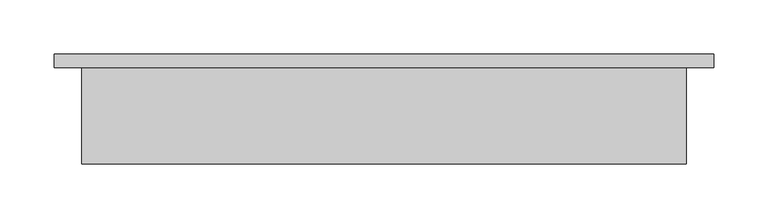
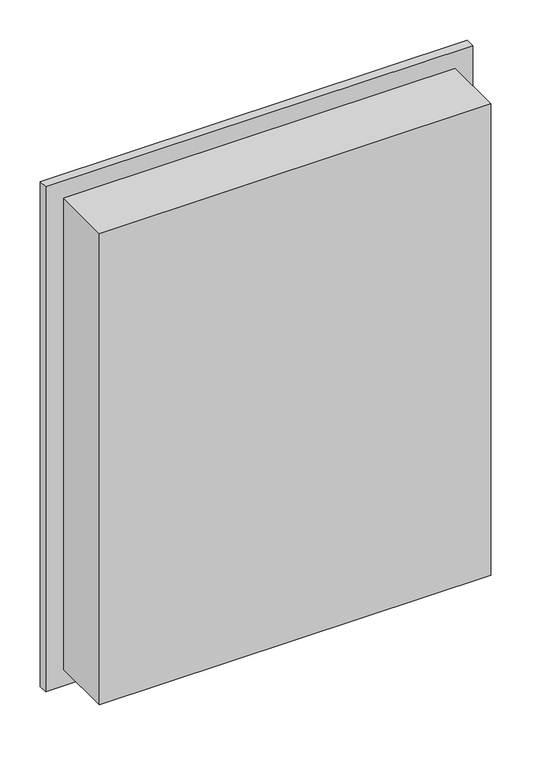
"""IFC4 building model written with IfcOpenShell, lengths in millimetres: furniture geometry, Medicine Cabinet, Recessed-NON-COLLECTUS : -."""

import ifcopenshell
import ifcopenshell.guid

model = None  # the IFC model being written
_history = None  # IfcOwnerHistory: only IFC2X3 demands one
_inside = {}  # id of a spatial element -> (the spatial element, [elements in it])
_under = {}  # id of a project, library or spatial element -> (it, [spatial elements below it])
_declared = {}  # id of a project -> (the project, [libraries it declares])
_typed = {}  # id of a type object -> (the type object, [elements of that type])
_made_of = {}  # id of a material, layer set ... -> (it, [elements and type objects made of it])


def new_model(schema):
    """Start an empty IFC model of exactly this schema.

    Asked for "IFC4X3", IfcOpenShell would pick the latest addendum, in which some entities
    have other attributes; the version numbers below select the first issue.
    IFC2X3 requires an IfcOwnerHistory on every rooted entity: one is made here for all.
    """
    global model, _history
    if schema == "IFC4X3":
        model = ifcopenshell.file(schema_version=(4, 3, 0, 0))
    else:
        model = ifcopenshell.file(schema=schema)
    _inside.clear()
    _under.clear()
    _declared.clear()
    _typed.clear()
    _made_of.clear()
    _history = None
    if model.schema == "IFC2X3":
        org = make("IfcOrganization", Name="unknown")
        user = make(
            "IfcPersonAndOrganization",
            ThePerson=make("IfcPerson", FamilyName="unknown"),
            TheOrganization=org,
        )
        app = make(
            "IfcApplication",
            ApplicationDeveloper=org,
            Version="unknown",
            ApplicationFullName="unknown",
            ApplicationIdentifier="unknown",
        )
        _history = make(
            "IfcOwnerHistory",
            OwningUser=user,
            OwningApplication=app,
            ChangeAction="ADDED",
            CreationDate=0,
        )
    return model


def make(cls, **values):
    """One entity of the class cls with the attributes given. An attribute that is None is left unset."""
    return model.create_entity(
        cls, **{name: value for name, value in values.items() if value is not None}
    )


def rooted(cls, **values):
    """An entity with a GlobalId (a new one), such as an element, a storey or a relation."""
    return make(cls, GlobalId=ifcopenshell.guid.new(), OwnerHistory=_history, **values)


def si_unit(unit_type, name, prefix=None):
    """IfcSIUnit, for example si_unit("LENGTHUNIT", "METRE", prefix="MILLI")."""
    return make("IfcSIUnit", UnitType=unit_type, Prefix=prefix, Name=name)


def assignment(units):
    """IfcUnitAssignment: the units of a project."""
    return None if units is None else make("IfcUnitAssignment", Units=units)


def point(xyz):
    """IfcCartesianPoint."""
    return None if xyz is None else make("IfcCartesianPoint", Coordinates=xyz)


def direction(xyz):
    """IfcDirection."""
    return None if xyz is None else make("IfcDirection", DirectionRatios=xyz)


def frame(location, z_axis=None, x_axis=None):
    """IfcAxis2Placement3D, a coordinate frame: its origin and axes. An axis left out is left unset."""
    return make(
        "IfcAxis2Placement3D",
        Location=point(location),
        Axis=direction(z_axis),
        RefDirection=direction(x_axis),
    )


def origin():
    """The frame at (0, 0, 0) with its axes left unset."""
    return frame((0.0, 0.0, 0.0))


def place(relative_to, where):
    """IfcLocalPlacement: puts the frame where relative to a parent placement (None: the world)."""
    return make(
        "IfcLocalPlacement", PlacementRelTo=relative_to, RelativePlacement=where
    )


def context(
    kind, dimensions, precision=None, world=None, true_north=None, identifier=None
):
    """IfcGeometricRepresentationContext, for example the 3D "Model" context."""
    return make(
        "IfcGeometricRepresentationContext",
        ContextIdentifier=identifier,
        ContextType=kind,
        CoordinateSpaceDimension=dimensions,
        Precision=precision,
        WorldCoordinateSystem=world,
        TrueNorth=true_north,
    )


def project(units=None, contexts=None):
    """IfcProject with its units and contexts."""
    return rooted(
        "IfcProject",
        Name="project",
        RepresentationContexts=contexts,
        UnitsInContext=assignment(units),
    )


def spatial(cls, under=None, at=None, **own):
    """A site, building, storey or space (cls), placed at a placement, below another one or the project."""
    s = rooted(cls, ObjectPlacement=at, **own)
    if under is not None:
        _under.setdefault(under.id(), (under, []))[1].append(s)
    return s


def polyline(points):
    """IfcPolyline through the points."""
    return make("IfcPolyline", Points=[point(p) for p in points])


def outline(outer, holes=None, kind="AREA"):
    """IfcArbitraryClosedProfileDef: a profile drawn as a closed curve; with holes, ...WithVoids."""
    if holes is None:
        return make("IfcArbitraryClosedProfileDef", ProfileType=kind, OuterCurve=outer)
    return make(
        "IfcArbitraryProfileDefWithVoids",
        ProfileType=kind,
        OuterCurve=outer,
        InnerCurves=holes,
    )


def extrude(swept, where, along, depth):
    """IfcExtrudedAreaSolid: the profile swept, set in the frame where, extruded along a direction by depth."""
    return make(
        "IfcExtrudedAreaSolid",
        SweptArea=swept,
        Position=where,
        ExtrudedDirection=direction(along),
        Depth=depth,
    )


def faces_of(points, faces, orient=None, outer=None):
    """IfcFace entities. A face is a list of loops; a loop is a list of indices into points, from 0.

    orient and outer hold one flag for each loop. By default every Orientation is true, the
    first loop of a face is its IfcFaceOuterBound and the others are IfcFaceBound.
    """
    made = []
    for i, loops in enumerate(faces):
        bounds = []
        for j, loop in enumerate(loops):
            is_outer = j == 0 if outer is None else outer[i][j]
            bounds.append(
                make(
                    "IfcFaceOuterBound" if is_outer else "IfcFaceBound",
                    Bound=make("IfcPolyLoop", Polygon=[points[k] for k in loop]),
                    Orientation=True if orient is None else orient[i][j],
                )
            )
        made.append(make("IfcFace", Bounds=bounds))
    return made


def faceted_brep(points, faces, orient=None, outer=None, voids=None):
    """IfcFacetedBrep: a solid bounded by flat faces; with voids (closed shells), ...WithVoids."""
    shared = [point(p) for p in points]
    hull = make("IfcClosedShell", CfsFaces=faces_of(shared, faces, orient, outer))
    if voids is None:
        return make("IfcFacetedBrep", Outer=hull)
    return make(
        "IfcFacetedBrepWithVoids",
        Outer=hull,
        Voids=[
            make(cls, CfsFaces=faces_of(shared, fs, o, b)) for cls, fs, o, b in voids
        ],
    )


def shape(context_of_items, identifier, shape_type, items):
    """IfcShapeRepresentation: the items that make up one representation, for example the "Body"."""
    return make(
        "IfcShapeRepresentation",
        ContextOfItems=context_of_items,
        RepresentationIdentifier=identifier,
        RepresentationType=shape_type,
        Items=items,
    )


def source(mapping_origin, context_of_items, identifier, shape_type, items):
    """IfcRepresentationMap: a shape defined once, which mapped items show again and again."""
    return make(
        "IfcRepresentationMap",
        MappingOrigin=mapping_origin,
        MappedRepresentation=shape(context_of_items, identifier, shape_type, items),
    )


def transform(
    local_origin,
    x_axis=None,
    y_axis=None,
    z_axis=None,
    scale=None,
    scale2=None,
    scale3=None,
    uniform=True,
):
    """IfcCartesianTransformationOperator3D, or its non-uniform kind. x_axis, y_axis, z_axis: its Axis1, 2, 3."""
    if uniform:
        return make(
            "IfcCartesianTransformationOperator3D",
            Axis1=direction(x_axis),
            Axis2=direction(y_axis),
            LocalOrigin=point(local_origin),
            Scale=scale,
            Axis3=direction(z_axis),
        )
    return make(
        "IfcCartesianTransformationOperator3DnonUniform",
        Axis1=direction(x_axis),
        Axis2=direction(y_axis),
        LocalOrigin=point(local_origin),
        Scale=scale,
        Axis3=direction(z_axis),
        Scale2=scale2,
        Scale3=scale3,
    )


def mapped(mapping_source, mapping_target):
    """IfcMappedItem: shows the shape of a source again, moved by a transform."""
    return make(
        "IfcMappedItem", MappingSource=mapping_source, MappingTarget=mapping_target
    )


def made_of(thing, what):
    """Note that an element or type object is made of a material, layer set ...; save() writes the relation."""
    if what is not None:
        _made_of.setdefault(what.id(), (what, []))[1].append(thing)
    return thing


def element(
    cls,
    number,
    at=None,
    inside=None,
    cuts=None,
    type_object=None,
    material=None,
    context=None,
    identifier="Body",
    shape_type=None,
    held_by="IfcProductDefinitionShape",
    body=None,
    shapes=None,
    **own,
):
    """One element of the class cls, such as IfcWall. Its Tag is "e" and its number.

    at: its placement. inside: the storey or other place that contains it. cuts: it is an
    opening in that element (IfcRelVoidsElement). A single representation is given by context,
    identifier, shape_type and body (its items); several are given by shapes. held_by: the class
    of the entity that holds the representations. save() writes the other relations.
    """
    e = rooted(cls, Tag="e%d" % number, ObjectPlacement=at, **own)
    if body is not None:
        shapes = [shape(context, identifier, shape_type, body)]
    if shapes is not None:
        e.Representation = make(held_by, Representations=shapes)
    if inside is not None:
        _inside.setdefault(inside.id(), (inside, []))[1].append(e)
    if cuts is not None:
        rooted(
            "IfcRelVoidsElement", RelatingBuildingElement=cuts, RelatedOpeningElement=e
        )
    if type_object is not None:
        _typed.setdefault(type_object.id(), (type_object, []))[1].append(e)
    return made_of(e, material)


def aggregate(whole, parts):
    """IfcRelAggregates: a whole, such as a stair, and the parts it consists of."""
    return rooted("IfcRelAggregates", RelatingObject=whole, RelatedObjects=parts)


def save(model, path):
    """Write the relations noted so far, then the file.

    IfcRelAggregates (storeys below a building ...), IfcRelContainedInSpatialStructure (elements
    in a storey), IfcRelDefinesByType, IfcRelAssociatesMaterial and IfcRelDeclares: one each for
    every whole, place, type object, material and project.
    """
    for whole, parts in _under.values():
        aggregate(whole, parts)
    for where, things in _inside.values():
        rooted(
            "IfcRelContainedInSpatialStructure",
            RelatedElements=things,
            RelatingStructure=where,
        )
    for kind, things in _typed.values():
        rooted("IfcRelDefinesByType", RelatedObjects=things, RelatingType=kind)
    for what, things in _made_of.values():
        rooted("IfcRelAssociatesMaterial", RelatedObjects=things, RelatingMaterial=what)
    for by, libraries in _declared.values():
        rooted("IfcRelDeclares", RelatingContext=by, RelatedDefinitions=libraries)
    model.write(path)


def furniture_f5e1b550(model_context):
    return source(origin(), model_context, "Body", "SolidModel", [
        faceted_brep([(609.6, 0.0, 762.0), (609.6, 0.0, 0.0), (0.0, 0.0, 0.0), (0.0, 0.0, 762.0), (596.9, 0.0, 12.7), (596.9, 0.0, 749.3), (12.7, 0.0, 749.3), (12.7, 0.0, 12.7), (609.6, -12.7, 762.0), (0.0, -12.7, 762.0), (0.0, -12.7, 0.0), (609.6, -12.7, 0.0), (12.7, -3.9310121, 12.7), (12.7, -3.9310121, 749.3), (596.9, -3.9310121, 749.3), (596.9, -3.9310121, 12.7)], [[[0, 1, 2, 3], [4, 5, 6, 7]], [[8, 9, 10, 11]], [[3, 9, 8, 0]], [[2, 10, 9, 3]], [[1, 11, 10, 2]], [[0, 8, 11, 1]], [[12, 13, 14, 15]], [[15, 4, 7, 12]], [[14, 5, 4, 15]], [[13, 6, 5, 14]], [[12, 7, 6, 13]]]),
        extrude(outline(polyline([(584.2, -12.7), (584.2, -101.6), (25.4, -101.6), (25.4, -12.7), (584.2, -12.7)])), frame((0.0, 0.0, 25.4), z_axis=(0.0, 0.0, 1.0), x_axis=(1.0, 0.0, 0.0)), (0.0, 0.0, 1.0), 711.2),
    ])


if __name__ == "__main__":
    model = new_model("IFC4")
    model_context = context("Model", 3, world=origin())
    ifc_project = project(units=[si_unit("LENGTHUNIT", "METRE", prefix="MILLI")], contexts=[model_context])
    site = spatial("IfcSite", under=ifc_project)
    building = spatial("IfcBuilding", under=site)
    placement = place(None, origin())
    furniture_shape = furniture_f5e1b550(model_context)
    element("IfcFurniture", 1, ObjectType="Medicine Cabinet, Recessed-NON-COLLECTUS : -", at=placement, inside=building, context=model_context, shape_type="MappedRepresentation", body=[
        mapped(furniture_shape, transform((0.0, 0.0, 0.0), x_axis=(1.0, 0.0, 0.0), y_axis=(0.0, 1.0, 0.0), z_axis=(0.0, 0.0, 1.0))),
    ])
    save(model, "model.ifc")

# Revit data of these elements
# Type "Medicine Cabinet, Recessed-NON-COLLECTUS : -"
#   External ID [instance default] = ""
#   Width = 609.6 mm
#   Height = 762 mm
#   Depth = 101.6 mm
#   Material = White
#   Default Elevation = 0
# Element 1 (IfcFurniture, "Medicine Cabinet, Recessed-NON-COLLECTUS : -")
#   Materials on its faces: "White"
# Materials
#   "White": class "Generic", colour RGB 255 255 255, transparency 0, Cost = 0
